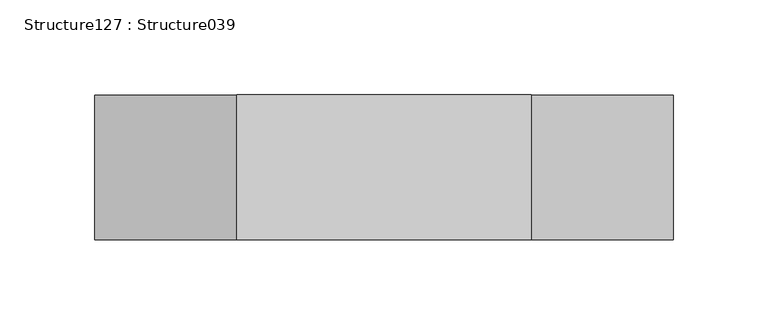
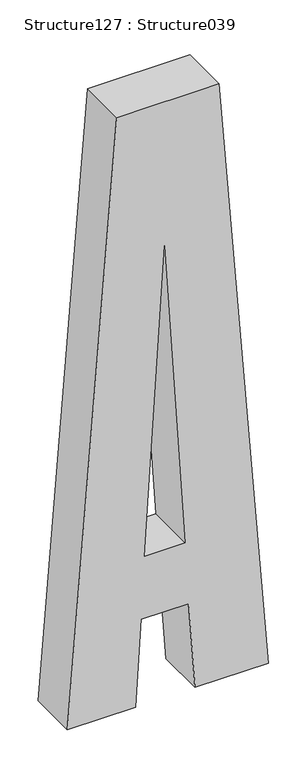
"""IFC4 building model written with IfcOpenShell, lengths in millimetres: proxy geometry, Structure127 : Structure039."""

from ifc_helpers import new_model, si_unit, frame, origin, place, context, project, spatial, polyline, outline, extrude, source, transform, mapped, element, save


def structure127_structure039_6851fcb4(model_context):
    return source(origin(), model_context, "Body", "SweptSolid", [
        extrude(outline(polyline([(3528.5825142, -48933.8172573), (3528.5825142, -48830.4663311), (3665.9109904, -48822.321317), (3665.9109904, -48750.2461614), (3528.5825142, -48740.717509), (3528.5825142, -48629.2272367), (4480.4419946, -48704.0073204), (4480.4419946, -48859.0277269), (3528.5825142, -48933.8172573)]), holes=[polyline([(3765.1859458, -48816.8743034), (4250.6490619, -48786.9532011), (3765.1859458, -48755.6862474), (3765.1859458, -48816.8743034)])]), frame((0.0, 247945.1599557, 0.0), z_axis=(0.0, 1.0, 0.0), x_axis=(0.0, 0.0, 1.0)), (0.0, 0.0, 1.0), 76.2),
    ])


if __name__ == "__main__":
    model = new_model("IFC4")
    model_context = context("Model", 3, world=origin())
    ifc_project = project(units=[si_unit("LENGTHUNIT", "METRE", prefix="MILLI")], contexts=[model_context])
    site = spatial("IfcSite", under=ifc_project)
    building = spatial("IfcBuilding", under=site)
    placement = place(None, origin())
    structure127_structure039_shape = structure127_structure039_6851fcb4(model_context)
    element("IfcBuildingElementProxy", 1, Name="Structure127 : Structure039", ObjectType="Structure127 : Structure039", at=placement, inside=building, context=model_context, shape_type="MappedRepresentation", body=[
        mapped(structure127_structure039_shape, transform((0.0, 0.0, 0.0), x_axis=(1.0, 0.0, 0.0), y_axis=(0.0, 1.0, 0.0), z_axis=(0.0, 0.0, 1.0))),
    ])
    save(model, "model.ifc")

# Revit data of these elements
# Type "Structure127 : Structure039"
#   NameOverride = "Structure039"
# Element 1 (IfcBuildingElementProxy, "Structure127 : Structure039")
#   Materials on its faces: "BRUSHED ALUM. LETTERING"
# Materials
#   "BRUSHED ALUM. LETTERING": class "Unassigned", colour RGB 169 181 186, transparency 0, Cost = 0
